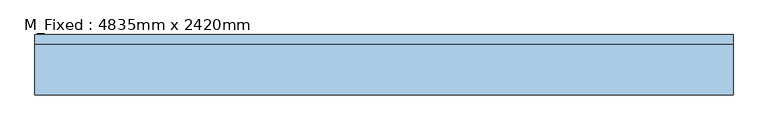
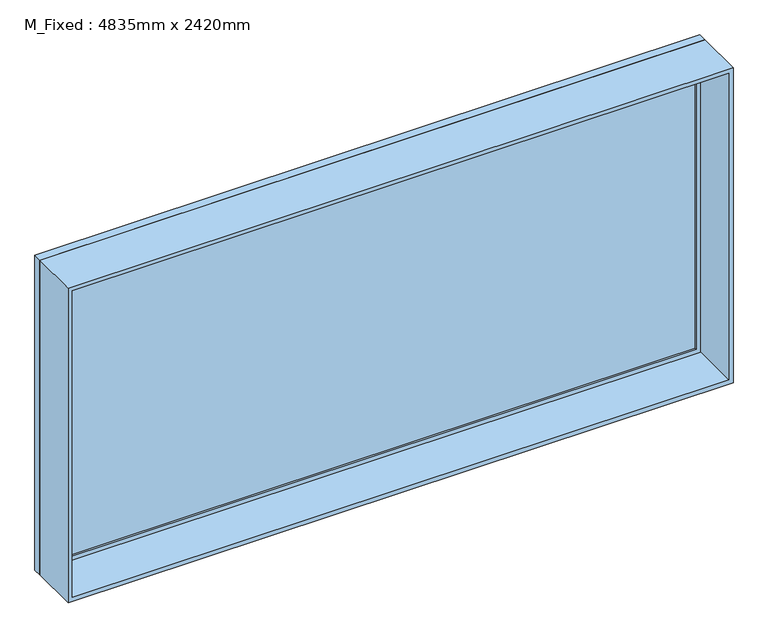
"""IFC4 building model written with IfcOpenShell, lengths in millimetres: window geometry, M_Fixed : 4835mm x 2420mm."""

from ifc_helpers import new_model, si_unit, frame, origin, place, context, project, spatial, polyline, outline, extrude, source, transform, mapped, element, save


def m_fixed_4835mm_x_2420mm_66b6dabf(model_context):
    return source(origin(), model_context, "Body", "SweptSolid", [
        extrude(outline(polyline([(-2354.5, 186.5), (2354.5, 186.5), (2354.5, 174.5), (-2354.5, 174.5), (-2354.5, 186.5)])), frame((0.0, 0.0, 163.0), z_axis=(0.0, 0.0, 1.0), x_axis=(1.0, 0.0, 0.0)), (0.0, 0.0, 1.0), 2294.0),
        extrude(outline(polyline([(2501.0, -2398.5), (119.0, -2398.5), (119.0, 2398.5), (2501.0, 2398.5), (2501.0, -2398.5)]), holes=[polyline([(2457.0, -2354.5), (2457.0, 2354.5), (163.0, 2354.5), (163.0, -2354.5), (2457.0, -2354.5)])]), frame((0.0, 158.5, 0.0), z_axis=(0.0, 1.0, 0.0), x_axis=(0.0, 0.0, 1.0)), (0.0, 0.0, 1.0), 44.0),
        extrude(outline(polyline([(2520.0, -2417.5), (100.0, -2417.5), (100.0, 2417.5), (2520.0, 2417.5), (2520.0, -2417.5)]), holes=[polyline([(2501.0, -2398.5), (2501.0, 2398.5), (119.0, 2398.5), (119.0, -2398.5), (2501.0, -2398.5)])]), frame((0.0, 158.5, 0.0), z_axis=(0.0, 1.0, 0.0), x_axis=(0.0, 0.0, 1.0)), (0.0, 0.0, 1.0), 63.0),
        extrude(outline(polyline([(2520.0, -2417.5), (100.0, -2417.5), (100.0, 2417.5), (2520.0, 2417.5), (2520.0, -2417.5)]), holes=[polyline([(2488.0, -2385.5), (2488.0, 2385.5), (132.0, 2385.5), (132.0, -2385.5), (2488.0, -2385.5)])]), frame((0.0, -195.5, 0.0), z_axis=(0.0, 1.0, 0.0), x_axis=(0.0, 0.0, 1.0)), (0.0, 0.0, 1.0), 354.0),
    ])


if __name__ == "__main__":
    model = new_model("IFC4")
    model_context = context("Model", 3, world=origin())
    ifc_project = project(units=[si_unit("LENGTHUNIT", "METRE", prefix="MILLI")], contexts=[model_context])
    site = spatial("IfcSite", under=ifc_project)
    building = spatial("IfcBuilding", under=site)
    placement = place(None, origin())
    m_fixed_4835mm_x_2420mm_shape = m_fixed_4835mm_x_2420mm_66b6dabf(model_context)
    element("IfcWindow", 1, ObjectType="M_Fixed : 4835mm x 2420mm", at=placement, inside=building, context=model_context, shape_type="MappedRepresentation", body=[
        mapped(m_fixed_4835mm_x_2420mm_shape, transform((0.0, 0.0, 0.0), x_axis=(1.0, 0.0, 0.0), y_axis=(0.0, 1.0, 0.0), z_axis=(0.0, 0.0, 1.0))),
    ])
    save(model, "model.ifc")

# Revit data of these elements
# Type "M_Fixed : 4835mm x 2420mm"
#   Manufacturer = "Manufacturer"
#   Type Mark = "05"
#   Construction Type = "Construction Type"
#   AccessibilityPerformance = "AccessibilityPerformance"
#   CodePerformance = "CodePerformance"
#   ConfigurationType = "ConfigurationType"
#   ConstructionType = "ConstructionType"
#   FireRating = "FireRating"
#   GlazingAreaFraction = "GlazingAreaFraction"
#   OperationType = "OperationType"
#   Area = "Area"
#   Color = "Color"
#   Constituents = "Constituents"
#   Features = "Features"
#   Finish = "Finish"
#   Grade = "Grade"
#   Material = "Material"
#   ModelReference = "ModelReference"
#   NominalHeight = "NominalHeight"
#   NominalLength = "NominalLength"
#   NominalWidth = "NominalWidth"
#   ProductionYear = "ProductionYear"
#   Reference = "Reference"
#   Shape = "Shape"
#   Size = "Size"
#   SustainabilityPerformance = "SustainabilityPerformance"
#   WarrantyDescription = "WarrantyDescription"
#   WarrantyDurationLabor = "WarrantyDurationLabor"
#   WarrantyDurationParts = "WarrantyDurationParts"
#   WarrantyGuarantorLabor = "WarrantyGuarantorLabor"
#   WarrantyGuarantorParts = "WarrantyGuarantorParts"
#   ExpectedLife = "ExpectedLife"
#   ReplacementCost = "ReplacementCost"
#   AssetAccountingType = "FIXED"
#   ModelLabel = "ModelLabel"
#   Height = 2.420 m
#   Default Sill Height = 0.100 m
#   Width = 4.835 m
#   Window Inset = 0.019 m
#   Frame Exterior Material = Sash
#   Frame Interior Material = Sash
#   Glass Pane Material = Glass
#   Sash = Sash
#   Wall Closure = (empty or 0)
# Element 1 (IfcWindow, "M_Fixed : 4835mm x 2420mm")
#   Materials on its faces: "Sash", "Glass"
# Materials
#   "Sash": class "Wood", colour RGB 224 178 126, transparency 0
#   "Glass": class "Glass", colour RGB 0 128 192, transparency 0.9
